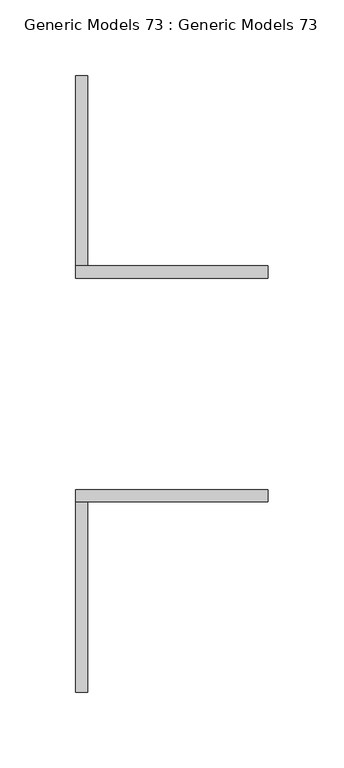
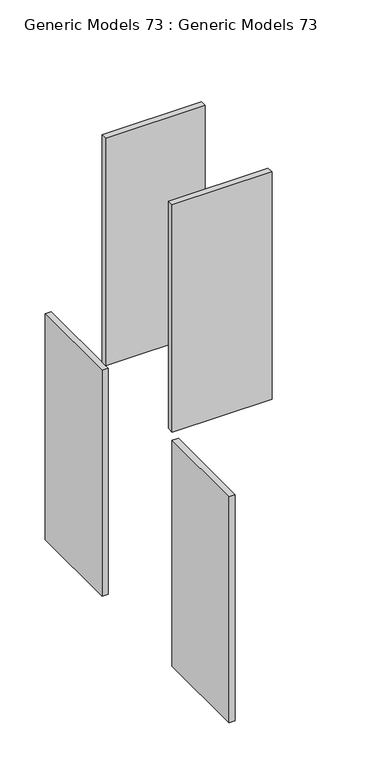
"""IFC4 building model written with IfcOpenShell, lengths in millimetres: proxy geometry, Generic Models 73 : Generic Models 73."""

from ifc_helpers import new_model, si_unit, frame, origin, place, context, project, spatial, polyline, outline, extrude, source, transform, mapped, element, save


def generic_models_73_generic_models_73_00176bc8(model_context):
    return source(origin(), model_context, "Body", "SweptSolid", [
        extrude(outline(polyline([(31923.0340778, 36329.6332942), (31930.9715778, 36329.6332942), (31930.9715778, 36204.2207942), (31923.0340778, 36204.2207942), (31923.0340778, 36329.6332942)])), frame((0.0, 0.0, 271481.55), z_axis=(0.0, 0.0, 1.0), x_axis=(1.0, 0.0, 0.0)), (0.0, 0.0, 1.0), 304.8),
        extrude(outline(polyline([(31923.0340778, 36610.6207942), (31930.9715778, 36610.6207942), (31930.9715778, 36485.2082942), (31923.0340778, 36485.2082942), (31923.0340778, 36610.6207942)])), frame((0.0, 0.0, 271481.55), z_axis=(0.0, 0.0, 1.0), x_axis=(1.0, 0.0, 0.0)), (0.0, 0.0, 1.0), 304.8),
        extrude(outline(polyline([(32050.0340778, 36485.2082942), (32050.0340778, 36477.2707942), (31923.0340778, 36477.2707942), (31923.0340778, 36485.2082942), (32050.0340778, 36485.2082942)])), frame((0.0, 0.0, 271797.4625), z_axis=(0.0, 0.0, 1.0), x_axis=(1.0, 0.0, 0.0)), (0.0, 0.0, 1.0), 306.5595065),
        extrude(outline(polyline([(32050.0340778, 36337.5707942), (32050.0340778, 36329.6332942), (31923.0340778, 36329.6332942), (31923.0340778, 36337.5707942), (32050.0340778, 36337.5707942)])), frame((0.0, 0.0, 271797.4625), z_axis=(0.0, 0.0, 1.0), x_axis=(1.0, 0.0, 0.0)), (0.0, 0.0, 1.0), 306.5595065),
    ])


if __name__ == "__main__":
    model = new_model("IFC4")
    model_context = context("Model", 3, world=origin())
    ifc_project = project(units=[si_unit("LENGTHUNIT", "METRE", prefix="MILLI")], contexts=[model_context])
    site = spatial("IfcSite", under=ifc_project)
    building = spatial("IfcBuilding", under=site)
    placement = place(None, origin())
    generic_models_73_generic_models_73_shape = generic_models_73_generic_models_73_00176bc8(model_context)
    element("IfcBuildingElementProxy", 1, Name="Generic Models 73 : Generic Models 73", ObjectType="Generic Models 73 : Generic Models 73", at=placement, inside=building, context=model_context, shape_type="MappedRepresentation", body=[
        mapped(generic_models_73_generic_models_73_shape, transform((0.0, 0.0, 0.0), x_axis=(1.0, 0.0, 0.0), y_axis=(0.0, 1.0, 0.0), z_axis=(0.0, 0.0, 1.0))),
    ])
    save(model, "model.ifc")

# Revit data of these elements
# Element 1 (IfcBuildingElementProxy, "Generic Models 73 : Generic Models 73")
#   Materials on its faces: "5/16\" THICK GALV. STEEL PLATE", "5/16 THICK GALV. SADDLE"
# Materials
#   "5/16\" THICK GALV. STEEL PLATE": class "Metal", colour RGB 199 199 199, transparency 0, Description = "Carbon steel", Cost = 0
#   "5/16 THICK GALV. SADDLE": class "Metal", colour RGB 199 199 199, transparency 0, Description = "Carbon steel", Cost = 0
